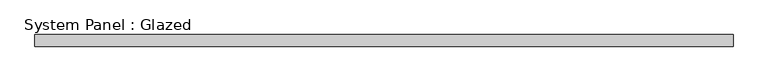
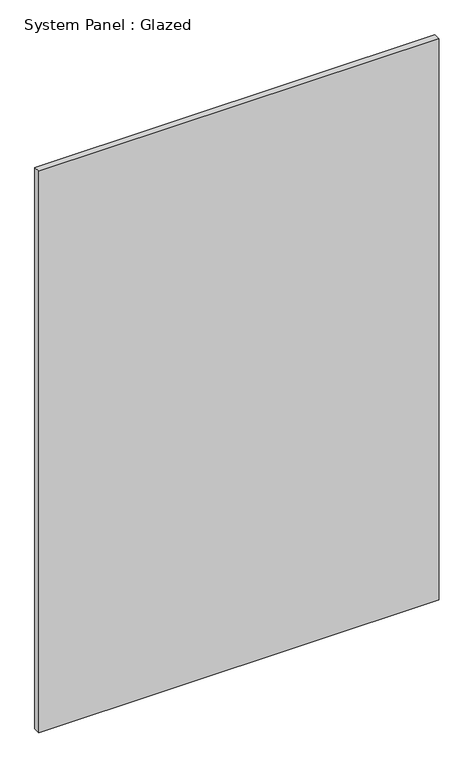
"""IFC4 building model written with IfcOpenShell, lengths in millimetres: plate geometry, System Panel : Glazed."""

import ifcopenshell
import ifcopenshell.guid

model = None  # the IFC model being written
_history = None  # IfcOwnerHistory: only IFC2X3 demands one
_inside = {}  # id of a spatial element -> (the spatial element, [elements in it])
_under = {}  # id of a project, library or spatial element -> (it, [spatial elements below it])
_declared = {}  # id of a project -> (the project, [libraries it declares])
_typed = {}  # id of a type object -> (the type object, [elements of that type])
_made_of = {}  # id of a material, layer set ... -> (it, [elements and type objects made of it])


def new_model(schema):
    """Start an empty IFC model of exactly this schema.

    Asked for "IFC4X3", IfcOpenShell would pick the latest addendum, in which some entities
    have other attributes; the version numbers below select the first issue.
    IFC2X3 requires an IfcOwnerHistory on every rooted entity: one is made here for all.
    """
    global model, _history
    if schema == "IFC4X3":
        model = ifcopenshell.file(schema_version=(4, 3, 0, 0))
    else:
        model = ifcopenshell.file(schema=schema)
    _inside.clear()
    _under.clear()
    _declared.clear()
    _typed.clear()
    _made_of.clear()
    _history = None
    if model.schema == "IFC2X3":
        org = make("IfcOrganization", Name="unknown")
        user = make(
            "IfcPersonAndOrganization",
            ThePerson=make("IfcPerson", FamilyName="unknown"),
            TheOrganization=org,
        )
        app = make(
            "IfcApplication",
            ApplicationDeveloper=org,
            Version="unknown",
            ApplicationFullName="unknown",
            ApplicationIdentifier="unknown",
        )
        _history = make(
            "IfcOwnerHistory",
            OwningUser=user,
            OwningApplication=app,
            ChangeAction="ADDED",
            CreationDate=0,
        )
    return model


def make(cls, **values):
    """One entity of the class cls with the attributes given. An attribute that is None is left unset."""
    return model.create_entity(
        cls, **{name: value for name, value in values.items() if value is not None}
    )


def rooted(cls, **values):
    """An entity with a GlobalId (a new one), such as an element, a storey or a relation."""
    return make(cls, GlobalId=ifcopenshell.guid.new(), OwnerHistory=_history, **values)


def si_unit(unit_type, name, prefix=None):
    """IfcSIUnit, for example si_unit("LENGTHUNIT", "METRE", prefix="MILLI")."""
    return make("IfcSIUnit", UnitType=unit_type, Prefix=prefix, Name=name)


def assignment(units):
    """IfcUnitAssignment: the units of a project."""
    return None if units is None else make("IfcUnitAssignment", Units=units)


def point(xyz):
    """IfcCartesianPoint."""
    return None if xyz is None else make("IfcCartesianPoint", Coordinates=xyz)


def direction(xyz):
    """IfcDirection."""
    return None if xyz is None else make("IfcDirection", DirectionRatios=xyz)


def frame(location, z_axis=None, x_axis=None):
    """IfcAxis2Placement3D, a coordinate frame: its origin and axes. An axis left out is left unset."""
    return make(
        "IfcAxis2Placement3D",
        Location=point(location),
        Axis=direction(z_axis),
        RefDirection=direction(x_axis),
    )


def origin():
    """The frame at (0, 0, 0) with its axes left unset."""
    return frame((0.0, 0.0, 0.0))


def origin_with_axes():
    """The frame at (0, 0, 0) with the z axis (0, 0, 1) and the x axis (1, 0, 0) written out."""
    return frame((0.0, 0.0, 0.0), z_axis=(0.0, 0.0, 1.0), x_axis=(1.0, 0.0, 0.0))


def place(relative_to, where):
    """IfcLocalPlacement: puts the frame where relative to a parent placement (None: the world)."""
    return make(
        "IfcLocalPlacement", PlacementRelTo=relative_to, RelativePlacement=where
    )


def context(
    kind, dimensions, precision=None, world=None, true_north=None, identifier=None
):
    """IfcGeometricRepresentationContext, for example the 3D "Model" context."""
    return make(
        "IfcGeometricRepresentationContext",
        ContextIdentifier=identifier,
        ContextType=kind,
        CoordinateSpaceDimension=dimensions,
        Precision=precision,
        WorldCoordinateSystem=world,
        TrueNorth=true_north,
    )


def project(units=None, contexts=None):
    """IfcProject with its units and contexts."""
    return rooted(
        "IfcProject",
        Name="project",
        RepresentationContexts=contexts,
        UnitsInContext=assignment(units),
    )


def spatial(cls, under=None, at=None, **own):
    """A site, building, storey or space (cls), placed at a placement, below another one or the project."""
    s = rooted(cls, ObjectPlacement=at, **own)
    if under is not None:
        _under.setdefault(under.id(), (under, []))[1].append(s)
    return s


def polyline(points):
    """IfcPolyline through the points."""
    return make("IfcPolyline", Points=[point(p) for p in points])


def outline(outer, holes=None, kind="AREA"):
    """IfcArbitraryClosedProfileDef: a profile drawn as a closed curve; with holes, ...WithVoids."""
    if holes is None:
        return make("IfcArbitraryClosedProfileDef", ProfileType=kind, OuterCurve=outer)
    return make(
        "IfcArbitraryProfileDefWithVoids",
        ProfileType=kind,
        OuterCurve=outer,
        InnerCurves=holes,
    )


def extrude(swept, where, along, depth):
    """IfcExtrudedAreaSolid: the profile swept, set in the frame where, extruded along a direction by depth."""
    return make(
        "IfcExtrudedAreaSolid",
        SweptArea=swept,
        Position=where,
        ExtrudedDirection=direction(along),
        Depth=depth,
    )


def shape(context_of_items, identifier, shape_type, items):
    """IfcShapeRepresentation: the items that make up one representation, for example the "Body"."""
    return make(
        "IfcShapeRepresentation",
        ContextOfItems=context_of_items,
        RepresentationIdentifier=identifier,
        RepresentationType=shape_type,
        Items=items,
    )


def source(mapping_origin, context_of_items, identifier, shape_type, items):
    """IfcRepresentationMap: a shape defined once, which mapped items show again and again."""
    return make(
        "IfcRepresentationMap",
        MappingOrigin=mapping_origin,
        MappedRepresentation=shape(context_of_items, identifier, shape_type, items),
    )


def transform(
    local_origin,
    x_axis=None,
    y_axis=None,
    z_axis=None,
    scale=None,
    scale2=None,
    scale3=None,
    uniform=True,
):
    """IfcCartesianTransformationOperator3D, or its non-uniform kind. x_axis, y_axis, z_axis: its Axis1, 2, 3."""
    if uniform:
        return make(
            "IfcCartesianTransformationOperator3D",
            Axis1=direction(x_axis),
            Axis2=direction(y_axis),
            LocalOrigin=point(local_origin),
            Scale=scale,
            Axis3=direction(z_axis),
        )
    return make(
        "IfcCartesianTransformationOperator3DnonUniform",
        Axis1=direction(x_axis),
        Axis2=direction(y_axis),
        LocalOrigin=point(local_origin),
        Scale=scale,
        Axis3=direction(z_axis),
        Scale2=scale2,
        Scale3=scale3,
    )


def mapped(mapping_source, mapping_target):
    """IfcMappedItem: shows the shape of a source again, moved by a transform."""
    return make(
        "IfcMappedItem", MappingSource=mapping_source, MappingTarget=mapping_target
    )


def made_of(thing, what):
    """Note that an element or type object is made of a material, layer set ...; save() writes the relation."""
    if what is not None:
        _made_of.setdefault(what.id(), (what, []))[1].append(thing)
    return thing


def element(
    cls,
    number,
    at=None,
    inside=None,
    cuts=None,
    type_object=None,
    material=None,
    context=None,
    identifier="Body",
    shape_type=None,
    held_by="IfcProductDefinitionShape",
    body=None,
    shapes=None,
    **own,
):
    """One element of the class cls, such as IfcWall. Its Tag is "e" and its number.

    at: its placement. inside: the storey or other place that contains it. cuts: it is an
    opening in that element (IfcRelVoidsElement). A single representation is given by context,
    identifier, shape_type and body (its items); several are given by shapes. held_by: the class
    of the entity that holds the representations. save() writes the other relations.
    """
    e = rooted(cls, Tag="e%d" % number, ObjectPlacement=at, **own)
    if body is not None:
        shapes = [shape(context, identifier, shape_type, body)]
    if shapes is not None:
        e.Representation = make(held_by, Representations=shapes)
    if inside is not None:
        _inside.setdefault(inside.id(), (inside, []))[1].append(e)
    if cuts is not None:
        rooted(
            "IfcRelVoidsElement", RelatingBuildingElement=cuts, RelatedOpeningElement=e
        )
    if type_object is not None:
        _typed.setdefault(type_object.id(), (type_object, []))[1].append(e)
    return made_of(e, material)


def aggregate(whole, parts):
    """IfcRelAggregates: a whole, such as a stair, and the parts it consists of."""
    return rooted("IfcRelAggregates", RelatingObject=whole, RelatedObjects=parts)


def save(model, path):
    """Write the relations noted so far, then the file.

    IfcRelAggregates (storeys below a building ...), IfcRelContainedInSpatialStructure (elements
    in a storey), IfcRelDefinesByType, IfcRelAssociatesMaterial and IfcRelDeclares: one each for
    every whole, place, type object, material and project.
    """
    for whole, parts in _under.values():
        aggregate(whole, parts)
    for where, things in _inside.values():
        rooted(
            "IfcRelContainedInSpatialStructure",
            RelatedElements=things,
            RelatingStructure=where,
        )
    for kind, things in _typed.values():
        rooted("IfcRelDefinesByType", RelatedObjects=things, RelatingType=kind)
    for what, things in _made_of.values():
        rooted("IfcRelAssociatesMaterial", RelatedObjects=things, RelatingMaterial=what)
    for by, libraries in _declared.values():
        rooted("IfcRelDeclares", RelatingContext=by, RelatedDefinitions=libraries)
    model.write(path)


def system_panel_glazed_8f795733(model_context):
    return source(origin(), model_context, "Body", "SweptSolid", [
        extrude(outline(polyline([(725.0514967, -49.5), (-725.0514967, -49.5), (-725.0514967, -24.5), (725.0514967, -24.5), (725.0514967, -49.5)])), origin_with_axes(), (0.0, 0.0, 1.0), 2150.0),
    ])


if __name__ == "__main__":
    model = new_model("IFC4")
    model_context = context("Model", 3, world=origin())
    ifc_project = project(units=[si_unit("LENGTHUNIT", "METRE", prefix="MILLI")], contexts=[model_context])
    site = spatial("IfcSite", under=ifc_project)
    building = spatial("IfcBuilding", under=site)
    placement = place(None, origin())
    system_panel_glazed_shape = system_panel_glazed_8f795733(model_context)
    element("IfcPlate", 1, ObjectType="System Panel : Glazed", at=placement, inside=building, context=model_context, shape_type="MappedRepresentation", body=[
        mapped(system_panel_glazed_shape, transform((0.0, 0.0, 0.0), x_axis=(1.0, 0.0, 0.0), y_axis=(0.0, 1.0, 0.0), z_axis=(0.0, 0.0, 1.0))),
    ])
    save(model, "model.ifc")

# Revit data of these elements
# Type "System Panel : Glazed"
#   Keynote = "H11"
#   Construction Type Id = "GSP4R"
#   Analytic Construction = "1/8 in Pilkington single glazing"
#   Visual Light Transmittance = 0.9
#   Solar Heat Gain Coefficient = 0.86
#   Heat Transfer Coefficient (U) = 6.7069 W/(m²·K)
# Element 1 (IfcPlate, "System Panel : Glazed")
#   Materials on its faces: "Glass"
# Materials
#   "Glass": class "Glass", colour RGB 0 128 192, transparency 0.9, Description = "Soda Lime Glass", Cost = 0
